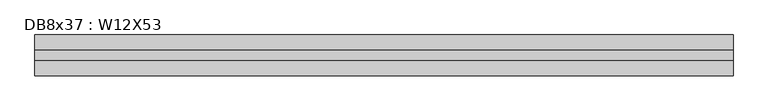
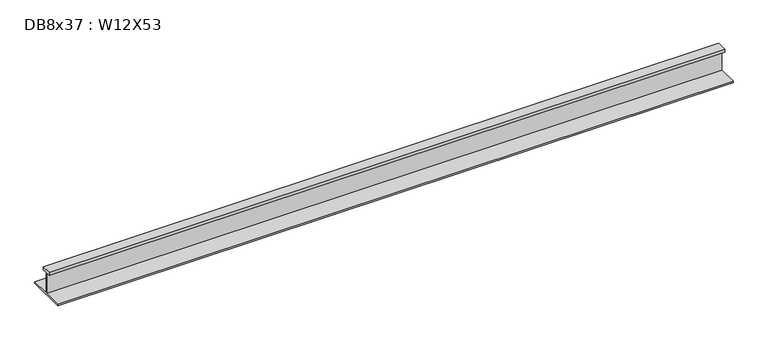
"""IFC4 building model written with IfcOpenShell, lengths in millimetres: beam geometry, DB8x37 : W12X53."""

import ifcopenshell
import ifcopenshell.guid

model = None  # the IFC model being written
_history = None  # IfcOwnerHistory: only IFC2X3 demands one
_inside = {}  # id of a spatial element -> (the spatial element, [elements in it])
_under = {}  # id of a project, library or spatial element -> (it, [spatial elements below it])
_declared = {}  # id of a project -> (the project, [libraries it declares])
_typed = {}  # id of a type object -> (the type object, [elements of that type])
_made_of = {}  # id of a material, layer set ... -> (it, [elements and type objects made of it])


def new_model(schema):
    """Start an empty IFC model of exactly this schema.

    Asked for "IFC4X3", IfcOpenShell would pick the latest addendum, in which some entities
    have other attributes; the version numbers below select the first issue.
    IFC2X3 requires an IfcOwnerHistory on every rooted entity: one is made here for all.
    """
    global model, _history
    if schema == "IFC4X3":
        model = ifcopenshell.file(schema_version=(4, 3, 0, 0))
    else:
        model = ifcopenshell.file(schema=schema)
    _inside.clear()
    _under.clear()
    _declared.clear()
    _typed.clear()
    _made_of.clear()
    _history = None
    if model.schema == "IFC2X3":
        org = make("IfcOrganization", Name="unknown")
        user = make(
            "IfcPersonAndOrganization",
            ThePerson=make("IfcPerson", FamilyName="unknown"),
            TheOrganization=org,
        )
        app = make(
            "IfcApplication",
            ApplicationDeveloper=org,
            Version="unknown",
            ApplicationFullName="unknown",
            ApplicationIdentifier="unknown",
        )
        _history = make(
            "IfcOwnerHistory",
            OwningUser=user,
            OwningApplication=app,
            ChangeAction="ADDED",
            CreationDate=0,
        )
    return model


def make(cls, **values):
    """One entity of the class cls with the attributes given. An attribute that is None is left unset."""
    return model.create_entity(
        cls, **{name: value for name, value in values.items() if value is not None}
    )


def rooted(cls, **values):
    """An entity with a GlobalId (a new one), such as an element, a storey or a relation."""
    return make(cls, GlobalId=ifcopenshell.guid.new(), OwnerHistory=_history, **values)


def si_unit(unit_type, name, prefix=None):
    """IfcSIUnit, for example si_unit("LENGTHUNIT", "METRE", prefix="MILLI")."""
    return make("IfcSIUnit", UnitType=unit_type, Prefix=prefix, Name=name)


def assignment(units):
    """IfcUnitAssignment: the units of a project."""
    return None if units is None else make("IfcUnitAssignment", Units=units)


def point(xyz):
    """IfcCartesianPoint."""
    return None if xyz is None else make("IfcCartesianPoint", Coordinates=xyz)


def direction(xyz):
    """IfcDirection."""
    return None if xyz is None else make("IfcDirection", DirectionRatios=xyz)


def frame(location, z_axis=None, x_axis=None):
    """IfcAxis2Placement3D, a coordinate frame: its origin and axes. An axis left out is left unset."""
    return make(
        "IfcAxis2Placement3D",
        Location=point(location),
        Axis=direction(z_axis),
        RefDirection=direction(x_axis),
    )


def origin():
    """The frame at (0, 0, 0) with its axes left unset."""
    return frame((0.0, 0.0, 0.0))


def place(relative_to, where):
    """IfcLocalPlacement: puts the frame where relative to a parent placement (None: the world)."""
    return make(
        "IfcLocalPlacement", PlacementRelTo=relative_to, RelativePlacement=where
    )


def context(
    kind, dimensions, precision=None, world=None, true_north=None, identifier=None
):
    """IfcGeometricRepresentationContext, for example the 3D "Model" context."""
    return make(
        "IfcGeometricRepresentationContext",
        ContextIdentifier=identifier,
        ContextType=kind,
        CoordinateSpaceDimension=dimensions,
        Precision=precision,
        WorldCoordinateSystem=world,
        TrueNorth=true_north,
    )


def project(units=None, contexts=None):
    """IfcProject with its units and contexts."""
    return rooted(
        "IfcProject",
        Name="project",
        RepresentationContexts=contexts,
        UnitsInContext=assignment(units),
    )


def spatial(cls, under=None, at=None, **own):
    """A site, building, storey or space (cls), placed at a placement, below another one or the project."""
    s = rooted(cls, ObjectPlacement=at, **own)
    if under is not None:
        _under.setdefault(under.id(), (under, []))[1].append(s)
    return s


def polyline(points):
    """IfcPolyline through the points."""
    return make("IfcPolyline", Points=[point(p) for p in points])


def outline(outer, holes=None, kind="AREA"):
    """IfcArbitraryClosedProfileDef: a profile drawn as a closed curve; with holes, ...WithVoids."""
    if holes is None:
        return make("IfcArbitraryClosedProfileDef", ProfileType=kind, OuterCurve=outer)
    return make(
        "IfcArbitraryProfileDefWithVoids",
        ProfileType=kind,
        OuterCurve=outer,
        InnerCurves=holes,
    )


def extrude(swept, where, along, depth):
    """IfcExtrudedAreaSolid: the profile swept, set in the frame where, extruded along a direction by depth."""
    return make(
        "IfcExtrudedAreaSolid",
        SweptArea=swept,
        Position=where,
        ExtrudedDirection=direction(along),
        Depth=depth,
    )


def shape(context_of_items, identifier, shape_type, items):
    """IfcShapeRepresentation: the items that make up one representation, for example the "Body"."""
    return make(
        "IfcShapeRepresentation",
        ContextOfItems=context_of_items,
        RepresentationIdentifier=identifier,
        RepresentationType=shape_type,
        Items=items,
    )


def source(mapping_origin, context_of_items, identifier, shape_type, items):
    """IfcRepresentationMap: a shape defined once, which mapped items show again and again."""
    return make(
        "IfcRepresentationMap",
        MappingOrigin=mapping_origin,
        MappedRepresentation=shape(context_of_items, identifier, shape_type, items),
    )


def transform(
    local_origin,
    x_axis=None,
    y_axis=None,
    z_axis=None,
    scale=None,
    scale2=None,
    scale3=None,
    uniform=True,
):
    """IfcCartesianTransformationOperator3D, or its non-uniform kind. x_axis, y_axis, z_axis: its Axis1, 2, 3."""
    if uniform:
        return make(
            "IfcCartesianTransformationOperator3D",
            Axis1=direction(x_axis),
            Axis2=direction(y_axis),
            LocalOrigin=point(local_origin),
            Scale=scale,
            Axis3=direction(z_axis),
        )
    return make(
        "IfcCartesianTransformationOperator3DnonUniform",
        Axis1=direction(x_axis),
        Axis2=direction(y_axis),
        LocalOrigin=point(local_origin),
        Scale=scale,
        Axis3=direction(z_axis),
        Scale2=scale2,
        Scale3=scale3,
    )


def mapped(mapping_source, mapping_target):
    """IfcMappedItem: shows the shape of a source again, moved by a transform."""
    return make(
        "IfcMappedItem", MappingSource=mapping_source, MappingTarget=mapping_target
    )


def made_of(thing, what):
    """Note that an element or type object is made of a material, layer set ...; save() writes the relation."""
    if what is not None:
        _made_of.setdefault(what.id(), (what, []))[1].append(thing)
    return thing


def element(
    cls,
    number,
    at=None,
    inside=None,
    cuts=None,
    type_object=None,
    material=None,
    context=None,
    identifier="Body",
    shape_type=None,
    held_by="IfcProductDefinitionShape",
    body=None,
    shapes=None,
    **own,
):
    """One element of the class cls, such as IfcWall. Its Tag is "e" and its number.

    at: its placement. inside: the storey or other place that contains it. cuts: it is an
    opening in that element (IfcRelVoidsElement). A single representation is given by context,
    identifier, shape_type and body (its items); several are given by shapes. held_by: the class
    of the entity that holds the representations. save() writes the other relations.
    """
    e = rooted(cls, Tag="e%d" % number, ObjectPlacement=at, **own)
    if body is not None:
        shapes = [shape(context, identifier, shape_type, body)]
    if shapes is not None:
        e.Representation = make(held_by, Representations=shapes)
    if inside is not None:
        _inside.setdefault(inside.id(), (inside, []))[1].append(e)
    if cuts is not None:
        rooted(
            "IfcRelVoidsElement", RelatingBuildingElement=cuts, RelatedOpeningElement=e
        )
    if type_object is not None:
        _typed.setdefault(type_object.id(), (type_object, []))[1].append(e)
    return made_of(e, material)


def aggregate(whole, parts):
    """IfcRelAggregates: a whole, such as a stair, and the parts it consists of."""
    return rooted("IfcRelAggregates", RelatingObject=whole, RelatedObjects=parts)


def save(model, path):
    """Write the relations noted so far, then the file.

    IfcRelAggregates (storeys below a building ...), IfcRelContainedInSpatialStructure (elements
    in a storey), IfcRelDefinesByType, IfcRelAssociatesMaterial and IfcRelDeclares: one each for
    every whole, place, type object, material and project.
    """
    for whole, parts in _under.values():
        aggregate(whole, parts)
    for where, things in _inside.values():
        rooted(
            "IfcRelContainedInSpatialStructure",
            RelatedElements=things,
            RelatingStructure=where,
        )
    for kind, things in _typed.values():
        rooted("IfcRelDefinesByType", RelatedObjects=things, RelatingType=kind)
    for what, things in _made_of.values():
        rooted("IfcRelAssociatesMaterial", RelatedObjects=things, RelatingMaterial=what)
    for by, libraries in _declared.values():
        rooted("IfcRelDeclares", RelatingContext=by, RelatedDefinitions=libraries)
    model.write(path)


def db8x37_w12x53_8bfe113e(model_context):
    return source(origin(), model_context, "Body", "SweptSolid", [
        extrude(outline(polyline([(38.1, 145.415), (38.1, 120.015), (2.921, 120.015), (2.921, -48.4505), (152.4, -48.4505), (152.4, -58.1025), (-152.4, -58.1025), (-152.4, -48.4505), (-2.921, -48.4505), (-2.921, 120.015), (-38.1, 120.015), (-38.1, 145.415), (38.1, 145.415)])), frame((-2604.516, 0.0, 0.0), z_axis=(1.0, 0.0, 0.0), x_axis=(0.0, 1.0, 0.0)), (0.0, 0.0, 1.0), 5211.445),
    ])


if __name__ == "__main__":
    model = new_model("IFC4")
    model_context = context("Model", 3, world=origin())
    ifc_project = project(units=[si_unit("LENGTHUNIT", "METRE", prefix="MILLI")], contexts=[model_context])
    site = spatial("IfcSite", under=ifc_project)
    building = spatial("IfcBuilding", under=site)
    placement = place(None, origin())
    db8x37_w12x53_shape = db8x37_w12x53_8bfe113e(model_context)
    element("IfcBeam", 1, ObjectType="DB8x37 : W12X53", at=placement, inside=building, context=model_context, shape_type="MappedRepresentation", body=[
        mapped(db8x37_w12x53_shape, transform((0.0, 0.0, 0.0), x_axis=(1.0, 0.0, 0.0), y_axis=(0.0, 1.0, 0.0), z_axis=(0.0, 0.0, 1.0))),
    ])
    save(model, "model.ifc")

# Revit data of these elements
# Type "DB8x37 : W12X53"
#   Assembly Code = "B10"
#   W = 53
#   Length [instance default] = 5' - 0"
#   bf = 0' - 10"
#   d = 1' - 0.1"
#   k = 0' - 1 3/8"
#   k2 = 0' - 0.8"
#   tf = 0' - 0.575"
#   tw = 0' - 0.345"
#   A = 0.108333 SF
#   Structural Material [instance default] = Steel ASTM A992
# Element 1 (IfcBeam, "DB8x37 : W12X53")
#   Materials on its faces: "Steel ASTM A992"
# Materials
#   "Steel ASTM A992": class "Metal", colour RGB 199 199 199, transparency 0, Description = "Structural steel 50ksi", Cost = 0
